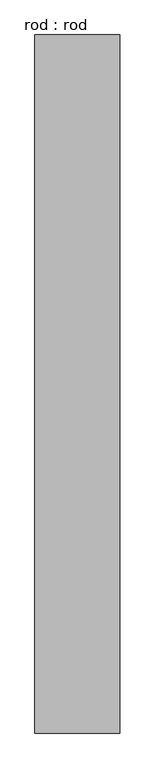
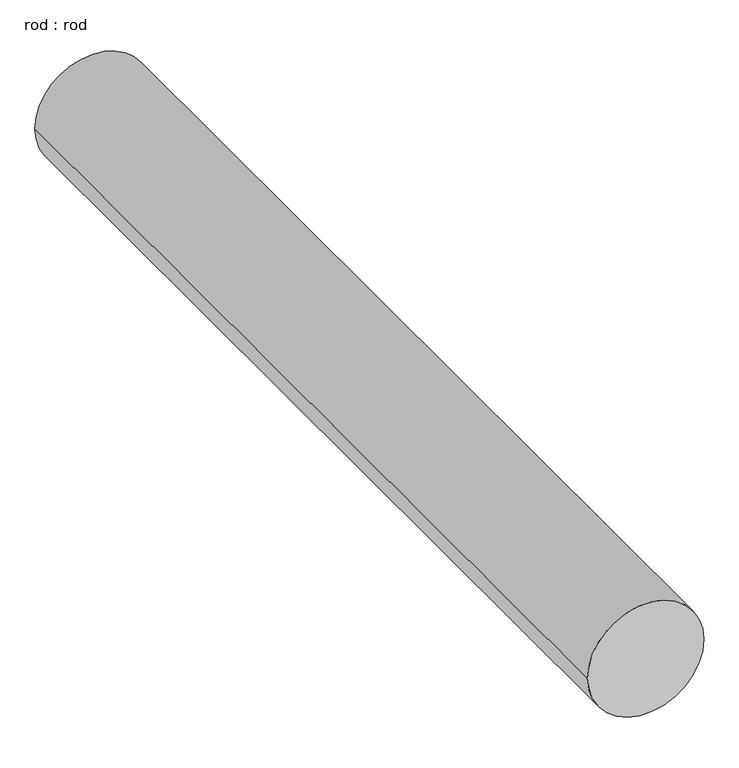
"""IFC4 building model written with IfcOpenShell, lengths in millimetres: proxy geometry, rod : rod."""

from ifc_helpers import new_model, si_unit, point, frame, frame_2d, origin, place, context, project, spatial, circle_curve, trimmed, segment, composite_curve, outline, extrude, source, transform, mapped, element, save


def rod_rod_8fe9abaa(model_context):
    return source(origin(), model_context, "Body", "SweptSolid", [
        extrude(outline(composite_curve([segment(trimmed(circle_curve(frame_2d((0.0108462, 0.0)), 200.0), [point((0.0108462, 200.0))], [point((0.0108462, -200.0))], False, "CARTESIAN"), True, "CONTINUOUS"), segment(trimmed(circle_curve(frame_2d((0.0108462, 0.0)), 200.0), [point((0.0108462, -200.0))], [point((0.0108462, 200.0))], False, "CARTESIAN"), True, "CONTINUOUS")], self_intersect=False)), frame((0.0, 2448.0857582, 0.0), z_axis=(0.0, 1.0, 0.0), x_axis=(0.0, 0.0, 1.0)), (0.0, 0.0, 1.0), 3289.2857143),
    ])


if __name__ == "__main__":
    model = new_model("IFC4")
    model_context = context("Model", 3, world=origin())
    ifc_project = project(units=[si_unit("LENGTHUNIT", "METRE", prefix="MILLI")], contexts=[model_context])
    site = spatial("IfcSite", under=ifc_project)
    building = spatial("IfcBuilding", under=site)
    placement = place(None, origin())
    rod_rod_shape = rod_rod_8fe9abaa(model_context)
    element("IfcBuildingElementProxy", 1, Name="rod : rod", ObjectType="rod : rod", at=placement, inside=building, context=model_context, shape_type="MappedRepresentation", body=[
        mapped(rod_rod_shape, transform((0.0, 0.0, 0.0), x_axis=(1.0, 0.0, 0.0), y_axis=(0.0, 1.0, 0.0), z_axis=(0.0, 0.0, 1.0))),
    ])
    save(model, "model.ifc")

# Revit data of these elements
# Type "rod : rod"
#   Default Elevation = 0
